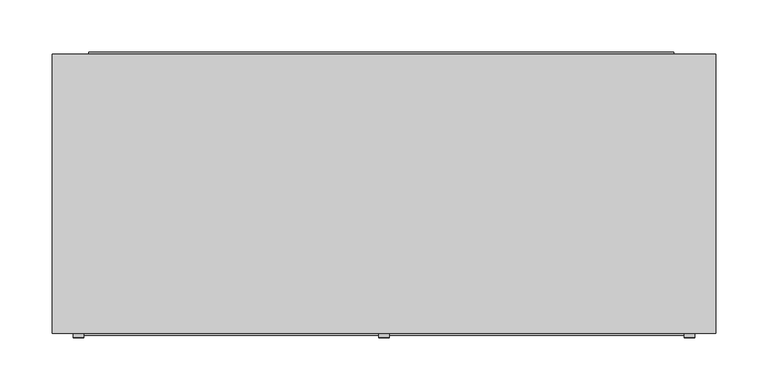
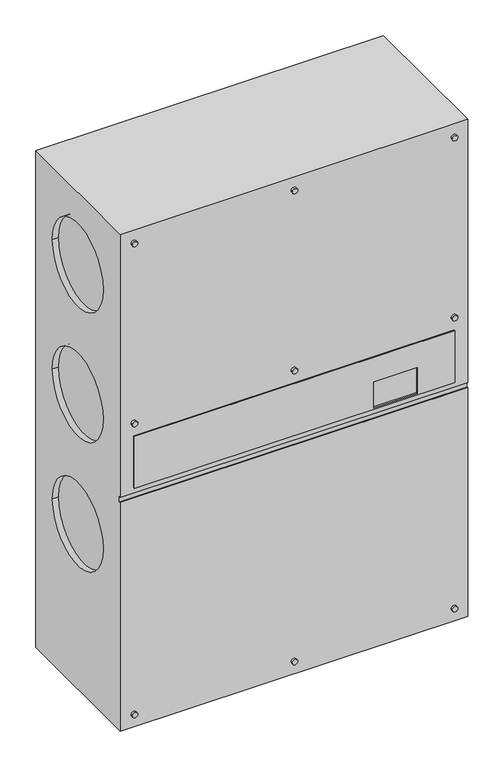
"""IFC4 building model written with IfcOpenShell, lengths in millimetres: proxy geometry, CPAC_WaterPumpControlCabinet : SONGROW INVERTER."""

from ifc_helpers import new_model, si_unit, point, frame, frame_2d, origin, place, context, project, spatial, polyline, circle_curve, trimmed, segment, composite_curve, outline, extrude, source, transform, mapped, element, save
from ifc_brep_helpers import plane_surface, revolved_surface, advanced_brep


def mechanical_equipment_97f4239b(model_context):
    return source(origin(), model_context, "Body", "SolidModel", [
        extrude(outline(composite_curve([segment(trimmed(circle_curve(frame_2d((25.0, 292.0)), 5.0), [point((25.0, 287.0))], [point((25.0, 297.0))], False, "CARTESIAN"), True, "CONTINUOUS"), segment(trimmed(circle_curve(frame_2d((25.0, 292.0)), 5.0), [point((25.0, 297.0))], [point((25.0, 287.0))], False, "CARTESIAN"), True, "CONTINUOUS")], self_intersect=False)), frame((0.0, -137.5, 0.0), z_axis=(0.0, 1.0, 0.0), x_axis=(0.0, 0.0, 1.0)), (0.0, 0.0, 1.0), 4.0),
        extrude(outline(composite_curve([segment(trimmed(circle_curve(frame_2d((25.0, 0.0)), 5.0), [point((25.0, -5.0))], [point((25.0, 5.0))], False, "CARTESIAN"), True, "CONTINUOUS"), segment(trimmed(circle_curve(frame_2d((25.0, 0.0)), 5.0), [point((25.0, 5.0))], [point((25.0, -5.0))], False, "CARTESIAN"), True, "CONTINUOUS")], self_intersect=False)), frame((0.0, -137.5, 0.0), z_axis=(0.0, 1.0, 0.0), x_axis=(0.0, 0.0, 1.0)), (0.0, 0.0, 1.0), 4.0),
        extrude(outline(composite_curve([segment(trimmed(circle_curve(frame_2d((25.0, -292.0)), 5.0), [point((25.0, -297.0))], [point((25.0, -287.0))], False, "CARTESIAN"), True, "CONTINUOUS"), segment(trimmed(circle_curve(frame_2d((25.0, -292.0)), 5.0), [point((25.0, -287.0))], [point((25.0, -297.0))], False, "CARTESIAN"), True, "CONTINUOUS")], self_intersect=False)), frame((0.0, -137.5, 0.0), z_axis=(0.0, 1.0, 0.0), x_axis=(0.0, 0.0, 1.0)), (0.0, 0.0, 1.0), 4.0),
        extrude(outline(composite_curve([segment(trimmed(circle_curve(frame_2d((586.7202987, 292.0)), 5.0), [point((586.7202987, 287.0))], [point((586.7202987, 297.0))], False, "CARTESIAN"), True, "CONTINUOUS"), segment(trimmed(circle_curve(frame_2d((586.7202987, 292.0)), 5.0), [point((586.7202987, 297.0))], [point((586.7202987, 287.0))], False, "CARTESIAN"), True, "CONTINUOUS")], self_intersect=False)), frame((0.0, -137.5, 0.0), z_axis=(0.0, 1.0, 0.0), x_axis=(0.0, 0.0, 1.0)), (0.0, 0.0, 1.0), 4.0),
        extrude(outline(composite_curve([segment(trimmed(circle_curve(frame_2d((586.7202987, 0.0)), 5.0), [point((586.7202987, -5.0))], [point((586.7202987, 5.0))], False, "CARTESIAN"), True, "CONTINUOUS"), segment(trimmed(circle_curve(frame_2d((586.7202987, 0.0)), 5.0), [point((586.7202987, 5.0))], [point((586.7202987, -5.0))], False, "CARTESIAN"), True, "CONTINUOUS")], self_intersect=False)), frame((0.0, -137.5, 0.0), z_axis=(0.0, 1.0, 0.0), x_axis=(0.0, 0.0, 1.0)), (0.0, 0.0, 1.0), 4.0),
        extrude(outline(composite_curve([segment(trimmed(circle_curve(frame_2d((586.7202987, -292.0)), 5.0), [point((586.7202987, -297.0))], [point((586.7202987, -287.0))], False, "CARTESIAN"), True, "CONTINUOUS"), segment(trimmed(circle_curve(frame_2d((586.7202987, -292.0)), 5.0), [point((586.7202987, -287.0))], [point((586.7202987, -297.0))], False, "CARTESIAN"), True, "CONTINUOUS")], self_intersect=False)), frame((0.0, -137.5, 0.0), z_axis=(0.0, 1.0, 0.0), x_axis=(0.0, 0.0, 1.0)), (0.0, 0.0, 1.0), 4.0),
        extrude(outline(composite_curve([segment(trimmed(circle_curve(frame_2d((934.0, 292.0)), 5.0), [point((934.0, 287.0))], [point((934.0, 297.0))], False, "CARTESIAN"), True, "CONTINUOUS"), segment(trimmed(circle_curve(frame_2d((934.0, 292.0)), 5.0), [point((934.0, 297.0))], [point((934.0, 287.0))], False, "CARTESIAN"), True, "CONTINUOUS")], self_intersect=False)), frame((0.0, -137.5, 0.0), z_axis=(0.0, 1.0, 0.0), x_axis=(0.0, 0.0, 1.0)), (0.0, 0.0, 1.0), 4.0),
        extrude(outline(composite_curve([segment(trimmed(circle_curve(frame_2d((934.0, 0.0)), 5.0), [point((934.0, -5.0))], [point((934.0, 5.0))], False, "CARTESIAN"), True, "CONTINUOUS"), segment(trimmed(circle_curve(frame_2d((934.0, 0.0)), 5.0), [point((934.0, 5.0))], [point((934.0, -5.0))], False, "CARTESIAN"), True, "CONTINUOUS")], self_intersect=False)), frame((0.0, -137.5, 0.0), z_axis=(0.0, 1.0, 0.0), x_axis=(0.0, 0.0, 1.0)), (0.0, 0.0, 1.0), 4.0),
        extrude(outline(composite_curve([segment(trimmed(circle_curve(frame_2d((934.0, -292.0)), 5.0), [point((934.0, -297.0))], [point((934.0, -287.0))], False, "CARTESIAN"), True, "CONTINUOUS"), segment(trimmed(circle_curve(frame_2d((934.0, -292.0)), 5.0), [point((934.0, -287.0))], [point((934.0, -297.0))], False, "CARTESIAN"), True, "CONTINUOUS")], self_intersect=False)), frame((0.0, -137.5, 0.0), z_axis=(0.0, 1.0, 0.0), x_axis=(0.0, 0.0, 1.0)), (0.0, 0.0, 1.0), 4.0),
        extrude(outline(polyline([(561.7202987, -292.0), (461.7202987, -292.0), (461.7202987, 292.0), (561.7202987, 292.0), (561.7202987, -292.0)]), holes=[polyline([(514.1545709, 224.4156239), (464.1545709, 224.4156239), (464.1545709, 144.4156239), (514.1545709, 144.4156239), (514.1545709, 224.4156239)])]), frame((0.0, -135.5, 0.0), z_axis=(0.0, 1.0, 0.0), x_axis=(0.0, 0.0, 1.0)), (0.0, 0.0, 1.0), 2.0),
        extrude(outline(polyline([(-281.9833812, 135.5), (277.0, 135.5), (277.0, 133.5), (-281.9833812, 133.5), (-281.9833812, 135.5)])), frame((0.0, 0.0, 31.8047247), z_axis=(0.0, 0.0, 1.0), x_axis=(1.0, 0.0, 0.0)), (0.0, 0.0, 1.0), 543.1143658),
        advanced_brep(
        [(-317.0, -133.5, 959.0), (317.0, -133.5, 959.0), (317.0, 133.5, 959.0), (-317.0, 133.5, 959.0), (-317.0, -133.5, 0.0), (-317.0, 133.5, 0.0), (317.0, 133.5, 0.0), (317.0, -133.5, 0.0), (-317.0, -133.5, 451.7202987), (317.0, -133.5, 451.7202987), (292.0, -133.5, 561.7202987), (292.0, -133.5, 461.7202987), (-292.0, -133.5, 461.7202987), (-292.0, -133.5, 561.7202987), (317.0, -133.5, 441.7202987), (-317.0, -133.5, 441.7202987), (317.0, -131.5, 451.7202987), (317.0, -131.5, 441.7202987), (317.0, 76.6555487, 687.4190905), (317.0, -75.3444513, 687.4190905), (317.0, -75.3444513, 707.4190905), (317.0, 76.6555487, 707.4190905), (317.0, 76.6555487, 812.4190905), (317.0, -75.3444513, 812.4190905), (317.0, -75.3444513, 832.4190905), (317.0, 76.6555487, 832.4190905), (-281.9833812, 133.5, 687.4190905), (277.0, 133.5, 687.4190905), (277.0, 133.5, 707.4190905), (-281.9833812, 133.5, 707.4190905), (-281.9833812, 133.5, 812.4190905), (277.0, 133.5, 812.4190905), (277.0, 133.5, 832.4190905), (-281.9833812, 133.5, 832.4190905), (-317.0, -131.5, 441.7202987), (-317.0, -131.5, 451.7202987), (-317.0, -80.0, 819.4595706), (-317.0, 80.0, 819.4595706), (-317.0, -80.0, 569.4595706), (-317.0, 80.0, 569.4595706), (-317.0, -80.0, 319.4595706), (-317.0, 80.0, 319.4595706), (292.0, -131.5, 561.7202987), (-292.0, -131.5, 561.7202987), (-292.0, -131.5, 461.7202987), (292.0, -131.5, 461.7202987), (315.0, 76.6555487, 687.4190905), (315.0, 76.6555487, 707.4190905), (315.0, -75.3444513, 707.4190905), (315.0, -75.3444513, 687.4190905), (315.0, 76.6555487, 812.4190905), (315.0, 76.6555487, 832.4190905), (315.0, -75.3444513, 832.4190905), (315.0, -75.3444513, 812.4190905), (-281.9833812, 131.5, 687.4190905), (-281.9833812, 131.5, 707.4190905), (277.0, 131.5, 707.4190905), (277.0, 131.5, 687.4190905), (-281.9833812, 131.5, 812.4190905), (-281.9833812, 131.5, 832.4190905), (277.0, 131.5, 832.4190905), (277.0, 131.5, 812.4190905), (-305.8411991, -80.0, 819.4595706), (-305.8411991, 80.0, 819.4595706), (-305.8411991, -80.0, 569.4595706), (-305.8411991, 80.0, 569.4595706), (-305.8411991, -80.0, 319.4595706), (-305.8411991, 80.0, 319.4595706)],
        [
            (0, 1),
            (1, 2),
            (2, 3),
            (3, 0),
            (4, 5),
            (5, 6),
            (6, 7),
            (7, 4),
            (0, 8),
            (8, 9),
            (9, 1),
            (10, 11),
            (11, 12),
            (12, 13),
            (13, 10),
            (7, 14),
            (14, 15),
            (15, 4),
            (9, 16),
            (16, 17),
            (17, 14),
            (6, 2),
            (18, 19),
            (19, 20),
            (20, 21),
            (21, 18),
            (22, 23),
            (23, 24),
            (24, 25),
            (25, 22),
            (5, 3),
            (26, 27),
            (27, 28),
            (28, 29),
            (29, 26),
            (30, 31),
            (31, 32),
            (32, 33),
            (33, 30),
            (15, 34),
            (34, 35),
            (35, 8),
            (36, 37, circle_curve(frame((-317.0, 0.0, 819.4595706), z_axis=(1.0, 0.0, 0.0), x_axis=(0.0, 1.0, 0.0)), 80.0)),
            (37, 36, circle_curve(frame((-317.0, 0.0, 819.4595706), z_axis=(1.0, 0.0, 0.0), x_axis=(0.0, 1.0, 0.0)), 80.0)),
            (38, 39, circle_curve(frame((-317.0, 0.0, 569.4595706), z_axis=(1.0, 0.0, 0.0), x_axis=(0.0, 1.0, 0.0)), 80.0)),
            (39, 38, circle_curve(frame((-317.0, 0.0, 569.4595706), z_axis=(1.0, 0.0, 0.0), x_axis=(0.0, 1.0, 0.0)), 80.0)),
            (40, 41, circle_curve(frame((-317.0, 0.0, 319.4595706), z_axis=(1.0, 0.0, 0.0), x_axis=(0.0, 1.0, 0.0)), 80.0)),
            (41, 40, circle_curve(frame((-317.0, 0.0, 319.4595706), z_axis=(1.0, 0.0, 0.0), x_axis=(0.0, 1.0, 0.0)), 80.0)),
            (42, 43),
            (43, 44),
            (44, 45),
            (45, 42),
            (45, 11),
            (10, 42),
            (44, 12),
            (43, 13),
            (46, 47),
            (47, 48),
            (48, 49),
            (49, 46),
            (49, 19),
            (18, 46),
            (48, 20),
            (47, 21),
            (50, 51),
            (51, 52),
            (52, 53),
            (53, 50),
            (53, 23),
            (22, 50),
            (52, 24),
            (51, 25),
            (54, 55),
            (55, 56),
            (56, 57),
            (57, 54),
            (57, 27),
            (26, 54),
            (56, 28),
            (55, 29),
            (58, 59),
            (59, 60),
            (60, 61),
            (61, 58),
            (61, 31),
            (30, 58),
            (60, 32),
            (59, 33),
            (34, 17),
            (16, 35),
            (62, 63, circle_curve(frame((-305.8411991, 0.0, 819.4595706), z_axis=(-1.0, 0.0, 0.0), x_axis=(0.0, 1.0, 0.0)), 80.0)),
            (63, 62, circle_curve(frame((-305.8411991, 0.0, 819.4595706), z_axis=(-1.0, 0.0, 0.0), x_axis=(0.0, 1.0, 0.0)), 80.0)),
            (63, 37),
            (36, 62),
            (64, 65, circle_curve(frame((-305.8411991, 0.0, 569.4595706), z_axis=(-1.0, 0.0, 0.0), x_axis=(0.0, 1.0, 0.0)), 80.0)),
            (65, 64, circle_curve(frame((-305.8411991, 0.0, 569.4595706), z_axis=(-1.0, 0.0, 0.0), x_axis=(0.0, 1.0, 0.0)), 80.0)),
            (65, 39),
            (38, 64),
            (66, 67, circle_curve(frame((-305.8411991, 0.0, 319.4595706), z_axis=(-1.0, 0.0, 0.0), x_axis=(0.0, 1.0, 0.0)), 80.0)),
            (67, 66, circle_curve(frame((-305.8411991, 0.0, 319.4595706), z_axis=(-1.0, 0.0, 0.0), x_axis=(0.0, 1.0, 0.0)), 80.0)),
            (67, 41),
            (40, 66),
        ],
        [
            plane_surface(frame((-317.0, -133.5, 959.0), z_axis=(0.0, 0.0, 1.0), x_axis=(1.0, 0.0, 0.0))),
            plane_surface(frame((-317.0, -133.5, 0.0), z_axis=(0.0, 0.0, -1.0), x_axis=(-1.0, 0.0, 0.0))),
            plane_surface(frame((-317.0, -133.5, 959.0), z_axis=(0.0, -1.0, 0.0), x_axis=(0.0, 0.0, -1.0))),
            plane_surface(frame((317.0, -133.5, 959.0), z_axis=(1.0, 0.0, 0.0), x_axis=(0.0, 0.0, -1.0))),
            plane_surface(frame((317.0, 133.5, 959.0), z_axis=(0.0, 1.0, 0.0), x_axis=(0.0, 0.0, -1.0))),
            plane_surface(frame((-317.0, 133.5, 959.0), z_axis=(-1.0, 0.0, 0.0), x_axis=(0.0, 0.0, -1.0))),
            plane_surface(frame((292.0, -131.5, 549.3886564), z_axis=(0.0, -1.0, 0.0), x_axis=(0.0, 0.0, -1.0))),
            plane_surface(frame((292.0, -131.5, 561.7202987), z_axis=(-1.0, 0.0, 0.0), x_axis=(0.0, -1.0, 0.0))),
            plane_surface(frame((292.0, -131.5, 461.7202987), z_axis=(0.0, 0.0, 1.0), x_axis=(0.0, -1.0, 0.0))),
            plane_surface(frame((-292.0, -131.5, 461.7202987), z_axis=(1.0, 0.0, 0.0), x_axis=(0.0, -1.0, 0.0))),
            plane_surface(frame((-292.0, -131.5, 561.7202987), z_axis=(0.0, 0.0, -1.0), x_axis=(0.0, -1.0, 0.0))),
            plane_surface(frame((315.0, -75.3444513, 687.4190905), z_axis=(1.0, 0.0, 0.0), x_axis=(0.0, -1.0, 0.0))),
            plane_surface(frame((315.0, 76.6555487, 687.4190905), z_axis=(0.0, 0.0, 1.0), x_axis=(1.0, 0.0, 0.0))),
            plane_surface(frame((315.0, -75.3444513, 687.4190905), z_axis=(0.0, 1.0, 0.0), x_axis=(1.0, 0.0, 0.0))),
            plane_surface(frame((315.0, -75.3444513, 707.4190905), z_axis=(0.0, 0.0, -1.0), x_axis=(1.0, 0.0, 0.0))),
            plane_surface(frame((315.0, 76.6555487, 707.4190905), z_axis=(0.0, -1.0, 0.0), x_axis=(1.0, 0.0, 0.0))),
            plane_surface(frame((315.0, -75.3444513, 812.4190905), z_axis=(1.0, 0.0, 0.0), x_axis=(0.0, -1.0, 0.0))),
            plane_surface(frame((315.0, 76.6555487, 812.4190905), z_axis=(0.0, 0.0, 1.0), x_axis=(1.0, 0.0, 0.0))),
            plane_surface(frame((315.0, -75.3444513, 812.4190905), z_axis=(0.0, 1.0, 0.0), x_axis=(1.0, 0.0, 0.0))),
            plane_surface(frame((315.0, -75.3444513, 832.4190905), z_axis=(0.0, 0.0, -1.0), x_axis=(1.0, 0.0, 0.0))),
            plane_surface(frame((315.0, 76.6555487, 832.4190905), z_axis=(0.0, -1.0, 0.0), x_axis=(1.0, 0.0, 0.0))),
            plane_surface(frame((277.0, 131.5, 687.4190905), z_axis=(0.0, 1.0, 0.0), x_axis=(1.0, 0.0, 0.0))),
            plane_surface(frame((-281.9833812, 131.5, 687.4190905), z_axis=(0.0, 0.0, 1.0), x_axis=(0.0, 1.0, 0.0))),
            plane_surface(frame((277.0, 131.5, 687.4190905), z_axis=(-1.0, 0.0, 0.0), x_axis=(0.0, 1.0, 0.0))),
            plane_surface(frame((277.0, 131.5, 707.4190905), z_axis=(0.0, 0.0, -1.0), x_axis=(0.0, 1.0, 0.0))),
            plane_surface(frame((-281.9833812, 131.5, 707.4190905), z_axis=(1.0, 0.0, 0.0), x_axis=(0.0, 1.0, 0.0))),
            plane_surface(frame((277.0, 131.5, 812.4190905), z_axis=(0.0, 1.0, 0.0), x_axis=(1.0, 0.0, 0.0))),
            plane_surface(frame((-281.9833812, 131.5, 812.4190905), z_axis=(0.0, 0.0, 1.0), x_axis=(0.0, 1.0, 0.0))),
            plane_surface(frame((277.0, 131.5, 812.4190905), z_axis=(-1.0, 0.0, 0.0), x_axis=(0.0, 1.0, 0.0))),
            plane_surface(frame((277.0, 131.5, 832.4190905), z_axis=(0.0, 0.0, -1.0), x_axis=(0.0, 1.0, 0.0))),
            plane_surface(frame((-281.9833812, 131.5, 832.4190905), z_axis=(1.0, 0.0, 0.0), x_axis=(0.0, 1.0, 0.0))),
            plane_surface(frame((-342.0, -131.5, 441.7202987), z_axis=(0.0, -1.0, 0.0), x_axis=(0.0, 0.0, 1.0))),
            plane_surface(frame((342.0, -131.5, 441.7202987), z_axis=(0.0, 0.0, 1.0), x_axis=(0.0, -1.0, 0.0))),
            plane_surface(frame((-342.0, -131.5, 451.7202987), z_axis=(0.0, 0.0, -1.0), x_axis=(0.0, -1.0, 0.0))),
            plane_surface(frame((-305.8411991, 80.0, 819.4595706), z_axis=(-1.0, 0.0, 0.0), x_axis=(0.0, 0.0, 1.0))),
            revolved_surface(polyline([(-305.8411991, 80.0, 819.4595706), (-317.0, 80.0, 819.4595706)]), (-317.0, 0.0, 819.4595706), (1.0, 0.0, 0.0)),
            plane_surface(frame((-305.8411991, 80.0, 569.4595706), z_axis=(-1.0, 0.0, 0.0), x_axis=(0.0, 0.0, 1.0))),
            revolved_surface(polyline([(-305.8411991, 80.0, 569.4595706), (-317.0, 80.0, 569.4595706)]), (-317.0, 0.0, 569.4595706), (1.0, 0.0, 0.0)),
            plane_surface(frame((-305.8411991, 80.0, 319.4595706), z_axis=(-1.0, 0.0, 0.0), x_axis=(0.0, 0.0, 1.0))),
            revolved_surface(polyline([(-305.8411991, 80.0, 319.4595706), (-317.0, 80.0, 319.4595706)]), (-317.0, 0.0, 319.4595706), (1.0, 0.0, 0.0)),
        ],
        [
            (0, [[1, 2, 3, 4]]),
            (1, [[5, 6, 7, 8]]),
            (2, [[-1, 9, 10, 11], [12, 13, 14, 15]]),
            (2, [[-8, 16, 17, 18]]),
            (3, [[-2, -11, 19, 20, 21, -16, -7, 22], [23, 24, 25, 26], [27, 28, 29, 30]]),
            (4, [[-3, -22, -6, 31], [32, 33, 34, 35], [36, 37, 38, 39]]),
            (5, [[-4, -31, -5, -18, 40, 41, 42, -9], [43, 44], [45, 46], [47, 48]]),
            (6, [[49, 50, 51, 52]]),
            (7, [[-52, 53, -12, 54]]),
            (8, [[-51, 55, -13, -53]]),
            (9, [[-50, 56, -14, -55]]),
            (10, [[-49, -54, -15, -56]]),
            (11, [[57, 58, 59, 60]]),
            (12, [[-60, 61, -23, 62]]),
            (13, [[-59, 63, -24, -61]]),
            (14, [[-58, 64, -25, -63]]),
            (15, [[-57, -62, -26, -64]]),
            (16, [[65, 66, 67, 68]]),
            (17, [[-68, 69, -27, 70]]),
            (18, [[-67, 71, -28, -69]]),
            (19, [[-66, 72, -29, -71]]),
            (20, [[-65, -70, -30, -72]]),
            (21, [[73, 74, 75, 76]]),
            (22, [[-76, 77, -32, 78]]),
            (23, [[-75, 79, -33, -77]]),
            (24, [[-74, 80, -34, -79]]),
            (25, [[-73, -78, -35, -80]]),
            (26, [[81, 82, 83, 84]]),
            (27, [[-84, 85, -36, 86]]),
            (28, [[-83, 87, -37, -85]]),
            (29, [[-82, 88, -38, -87]]),
            (30, [[-81, -86, -39, -88]]),
            (31, [[89, -20, 90, -41]]),
            (32, [[-89, -40, -17, -21]]),
            (33, [[-90, -19, -10, -42]]),
            (34, [[91, 92]]),
            (35, [[-92, 93, -43, 94]]),
            (35, [[-91, -94, -44, -93]]),
            (36, [[95, 96]]),
            (37, [[-96, 97, -45, 98]]),
            (37, [[-95, -98, -46, -97]]),
            (38, [[99, 100]]),
            (39, [[-100, 101, -47, 102]]),
            (39, [[-99, -102, -48, -101]]),
        ],
    ),
    ])


if __name__ == "__main__":
    model = new_model("IFC4")
    model_context = context("Model", 3, world=origin())
    ifc_project = project(units=[si_unit("LENGTHUNIT", "METRE", prefix="MILLI")], contexts=[model_context])
    site = spatial("IfcSite", under=ifc_project)
    building = spatial("IfcBuilding", under=site)
    placement = place(None, origin())
    mechanical_equipment_shape = mechanical_equipment_97f4239b(model_context)
    element("IfcBuildingElementProxy", 1, Name="CPAC_WaterPumpControlCabinet : SONGROW INVERTER", ObjectType="CPAC_WaterPumpControlCabinet : SONGROW INVERTER", at=placement, inside=building, context=model_context, shape_type="MappedRepresentation", body=[
        mapped(mechanical_equipment_shape, transform((0.0, 0.0, 0.0), x_axis=(1.0, 0.0, 0.0), y_axis=(0.0, 1.0, 0.0), z_axis=(0.0, 0.0, 1.0))),
    ])
    save(model, "model.ifc")

# Revit data of these elements
# Type "CPAC_WaterPumpControlCabinet : SONGROW INVERTER"
#   Weight Net (Kg) = "215"
#   Uniformat II Description = ""
#   Uniformat II Code = ""
#   Uniclass 2015 Name = ""
#   Uniclass 2015 Code = ""
#   Uniclass 2.0 Description = ""
#   Uniclass 2.0 Code = ""
#   Uniclass 1.4 Description = ""
#   Uniclass 1.4 Code = ""
#   URL = "http://partner.lge.com/global"
#   UNSPSC Code = "40101701"
#   Type = ""
#   Temp Operating Range (Heating)(F) = ""
#   Temp Operating Range (Heating)(C) = ""
#   Temp Operating Range (Cooling)(F) = ""
#   Temp Operating Range (Cooling)(C) = ""
#   Technical description = ""
#   Sound Pressure Level Heating (dB(A)) = ""
#   Sound Pressure Level Cooling (dB(A)) = ""
#   Refrigerant Type = ""
#   Refrigerant Charge (lbs) = ""
#   Refrigerant Charge (kg) = ""
#   Product certification = ""
#   Product Guid = "fbfb564d-6f3d-44f8-af9b-1278b1d9e006"
#   Price = "8000 THB/unit"
#   Power Supply (Ph_V_Hz) = ""
#   Power Input (Heating)(kW) = ""
#   Power Input (Cooling)(kW) = ""
#   Pipe Connection_Low Gas Side (Heat Recovery)(mm) = ""
#   Pipe Connection_Low Gas Side (Heat Recovery)(inch) = ""
#   Pipe Connection_Liquid Side (mm) = ""
#   Pipe Connection_Liquid Side (inch) = ""
#   Pipe Connection_High Gas Side (Heat Recovery)(mm) = ""
#   Pipe Connection_High Gas Side (Heat Recovery)(inch) = ""
#   Pipe Connection_Gas Side (mm) = ""
#   Pipe Connection_Gas Side (inch) = ""
#   OmniClass Description = ""
#   OmniClass Code = ""
#   Net Weight (lbs) = ""
#   Net Weight (kg) = ""
#   NBS Reference Description = "Air Conditioning Systems"
#   NBS Reference Code = "65-80-05"
#   Model name = ""
#   Material secondary = "Copper"
#   Material main = "Steel"
#   Masterformat 2014 Description = ""
#   Masterformat 2014 Code = ""
#   Manufacturer = "LG Electronics"
#   MCA (A) = ""
#   Installation instructions = ""
#   Indoor Unit Total Capacity = ""
#   Indoor Unit Model Max Quantity = ""
#   Independent Unit = ""
#   IFC Classification = "Air Terminal"
#   Heating Capacity (kW) = ""
#   Heating Capacity (Btu/h) = ""
#   Fan Type = ""
#   Fan Motor Output (kW) = ""
#   Fan Air Flow Rate (CMM) = ""
#   Fan Air Flow Rate (CFM) = ""
#   EAN code = ""
#   Dimensions (WxHxD)(mm) = ""
#   Dimensions (WxHxD)(inch) = ""
#   Date of publishing = ""
#   Cooling Capacity (kW) = ""
#   Cooling Capacity (Btu/h) = ""
#   Compressor Type = ""
#   Communication Cable (mm2) = ""
#   Chassis name = ""
#   COBIe Type Category = ""
#   BIMobject main category code = "hvac"
#   BIMobject main category = "HVAC"
#   BIMobject category code = "hvac-air-con"
#   BIMobject category = "Air Conditioning"
#   Width offset bottom = 0' - 2.55906"
#   Width = 0' - 10.51181"
#   Right offset top = 0' - 11.14173"
#   Right offset front = 0' - 8.26772"
#   Right offset size = 0' - 3.50394"
#   Refrigerant Low Gas Connection Radius = 0.37598"
#   Refrigerant High Gas Connection Radius = 0.31299"
#   Refrigerant Low Gas Connection Offset Top = 0' - 8.8189"
#   Refrigerant Low Gas Connection Offset Front = 0' - 10.07874"
#   Refrigerant Low Gas Connection Diameter = 0.75197"
#   Refrigerant Liquid Connection Radius = 0.18701"
#   Refrigerant Liquid Connection Offset Top = 0' - 8.8189"
#   Refrigerant Liquid Connection Offset Front = 0' - 8.14961"
#   Refrigerant Liquid Connection Diameter = 0.37402"
#   Refrigerant High Gas Connection Diameter = 0.62598"
#   Length = 2' - 0.96063"
#   Height offset top = 0' - 3.14961"
#   Height offset mid = 2' - 6.86614"
#   Height offset front top = 0' - 1.53543"
#   Height offset front bottom = 2' - 1.35433"
#   Height offset bottom = 0' - 3.74016"
#   Height = 3' - 1.75591"
#   Fan offset side = 0' - 3.93701"
#   Fan offset right left = 0' - 8.46457"
#   Fan offset mid = 0' - 11.69291"
#   Fan offset front width = 0' - 2.59843"
#   Fan offset front side = 0' - 1.22047"
#   Fan offset front = 0' - 0.90551"
#   Fan offset circle radius = 0' - 1.9685"
#   Fan offset center = 0' - 11.88976"
#   Fan offset back = 0' - 0.90551"
#   Edition number = 1
#   Clearance Zone = yes
#   Default Elevation = 0
# Element 1 (IfcBuildingElementProxy, "CPAC_WaterPumpControlCabinet : SONGROW INVERTER")
#   Materials on its faces: "LG Paint-1"
# Materials
#   "LG Paint-1": class "Miscellaneous", colour RGB 200 200 200, transparency 0
